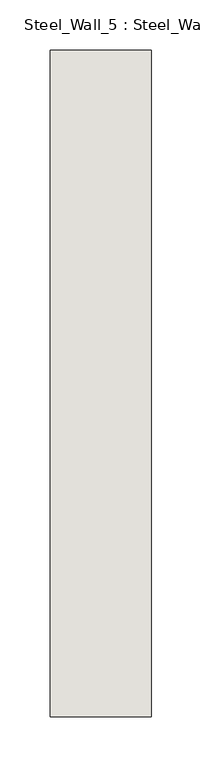
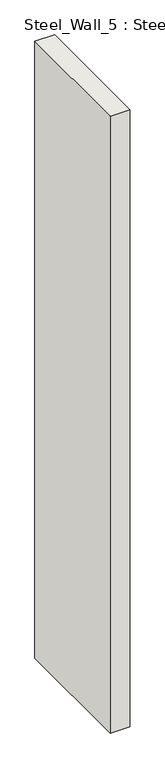
"""IFC4 building model written with IfcOpenShell, lengths in millimetres: wall geometry, Steel_Wall_5 : Steel_Wall_5."""

from ifc_helpers import new_model, si_unit, frame, origin, place, context, project, spatial, polyline, outline, extrude, source, transform, mapped, element, save


def steel_wall_5_steel_wall_5_69cba077(model_context):
    return source(origin(), model_context, "Body", "SweptSolid", [
        extrude(outline(polyline([(215.0, 16755.0), (215.0, 16095.0), (115.0, 16095.0), (115.0, 16755.0), (215.0, 16755.0)])), frame((0.0, 0.0, 250.0), z_axis=(0.0, 0.0, 1.0), x_axis=(1.0, 0.0, 0.0)), (0.0, 0.0, 1.0), 3300.0),
    ])


if __name__ == "__main__":
    model = new_model("IFC4")
    model_context = context("Model", 3, world=origin())
    ifc_project = project(units=[si_unit("LENGTHUNIT", "METRE", prefix="MILLI")], contexts=[model_context])
    site = spatial("IfcSite", under=ifc_project)
    building = spatial("IfcBuilding", under=site)
    placement = place(None, origin())
    steel_wall_5_steel_wall_5_shape = steel_wall_5_steel_wall_5_69cba077(model_context)
    element("IfcWall", 1, ObjectType="Steel_Wall_5 : Steel_Wall_5", at=placement, inside=building, context=model_context, shape_type="MappedRepresentation", body=[
        mapped(steel_wall_5_steel_wall_5_shape, transform((0.0, 0.0, 0.0), x_axis=(1.0, 0.0, 0.0), y_axis=(0.0, 1.0, 0.0), z_axis=(0.0, 0.0, 1.0))),
    ])
    save(model, "model.ifc")

# Revit data of these elements
# Type "Steel_Wall_5 : Steel_Wall_5"
#   NameOverride = "Steel_Wall_5"
# Element 1 (IfcWall, "Steel_Wall_5 : Steel_Wall_5")
#   Materials on its faces: "IfcSurfaceStyle #33"
# Materials
#   "IfcSurfaceStyle #33": class "Unassigned", colour RGB 214 214 214, transparency 0
